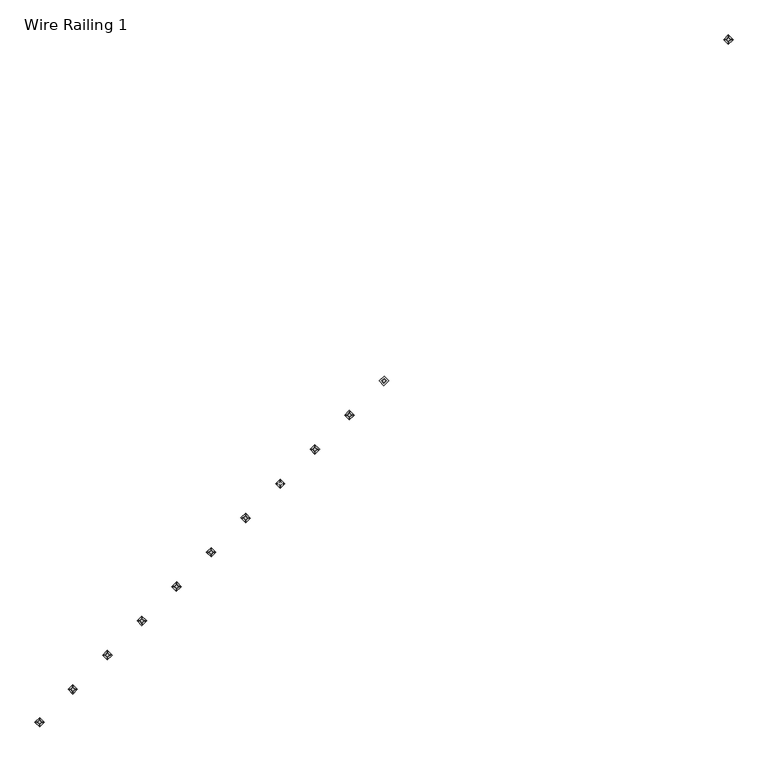
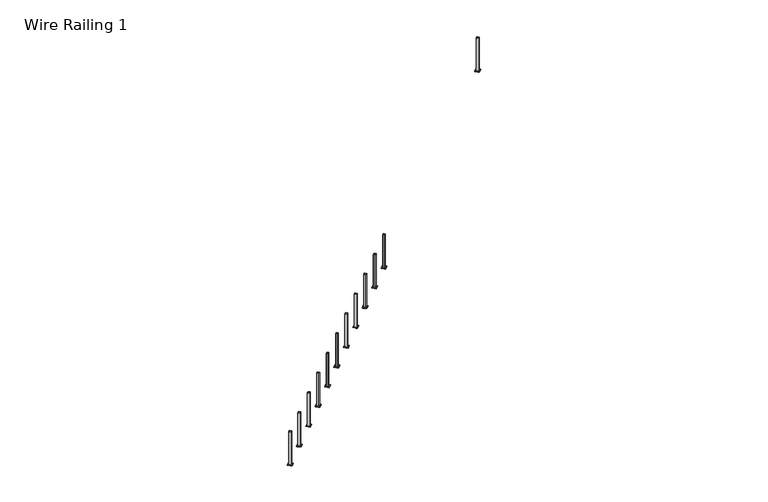
"""IFC4 building model written with IfcOpenShell, lengths in millimetres: railing geometry, Wire Railing 1."""

from ifc_helpers import new_model, si_unit, point, frame, frame_2d, origin, place, context, project, spatial, polyline, circle_curve, trimmed, segment, composite_curve, outline, extrude, source, transform, mapped, element, save


def wire_railing_1_32efedd6(model_context):
    return source(origin(), model_context, "Body", "SweptSolid", [
        extrude(outline(polyline([(39073.6633183, 30885.6288927), (39163.8685639, 30975.0269557), (39253.2666269, 30884.82171), (39163.0613812, 30795.4236471), (39073.6633183, 30885.6288927)])), frame((0.0, 0.0, 263956.8), z_axis=(0.0, 0.0, 1.0), x_axis=(1.0, 0.0, 0.0)), (0.0, 0.0, 1.0), 6.35),
        extrude(outline(polyline([(39120.8091868, 30885.4170073), (39163.6566785, 30927.8810871), (39206.1207584, 30885.0335955), (39163.2732667, 30842.5695156), (39120.8091868, 30885.4170073)]), holes=[polyline([(39129.7893522, 30885.3766481), (39163.3136258, 30851.549681), (39197.1405929, 30885.0739546), (39163.6163193, 30918.9009217), (39129.7893522, 30885.3766481)])]), frame((0.0, 0.0, 263956.8), z_axis=(0.0, 0.0, 1.0), x_axis=(1.0, 0.0, 0.0)), (0.0, 0.0, 1.0), 1047.75),
        extrude(outline(composite_curve([segment(trimmed(circle_curve(frame_2d((38502.5370002, 30167.6303323)), 6.35), [point((38507.0069034, 30163.12007))], [point((38498.0670971, 30172.1405946))], False, "CARTESIAN"), True, "CONTINUOUS"), segment(trimmed(circle_curve(frame_2d((38502.5370002, 30167.6303323)), 6.35), [point((38498.0670971, 30172.1405946))], [point((38507.0069034, 30163.12007))], False, "CARTESIAN"), True, "CONTINUOUS")], self_intersect=False)), frame((0.0, 0.0, 263956.8), z_axis=(0.0, 0.0, 1.0), x_axis=(1.0, 0.0, 0.0)), (0.0, 0.0, 1.0), 12.7),
        extrude(outline(composite_curve([segment(trimmed(circle_curve(frame_2d((38439.9583562, 30230.7740042)), 6.35), [point((38444.4282593, 30226.263742))], [point((38435.488453, 30235.2842665))], False, "CARTESIAN"), True, "CONTINUOUS"), segment(trimmed(circle_curve(frame_2d((38439.9583562, 30230.7740042)), 6.35), [point((38435.488453, 30235.2842665))], [point((38444.4282593, 30226.263742))], False, "CARTESIAN"), True, "CONTINUOUS")], self_intersect=False)), frame((0.0, 0.0, 263956.8), z_axis=(0.0, 0.0, 1.0), x_axis=(1.0, 0.0, 0.0)), (0.0, 0.0, 1.0), 12.7),
        extrude(outline(composite_curve([segment(trimmed(circle_curve(frame_2d((38565.6806722, 30230.2089763)), 6.35), [point((38570.1505753, 30225.6987141))], [point((38561.210769, 30234.7192386))], False, "CARTESIAN"), True, "CONTINUOUS"), segment(trimmed(circle_curve(frame_2d((38565.6806722, 30230.2089763)), 6.35), [point((38561.210769, 30234.7192386))], [point((38570.1505753, 30225.6987141))], False, "CARTESIAN"), True, "CONTINUOUS")], self_intersect=False)), frame((0.0, 0.0, 263956.8), z_axis=(0.0, 0.0, 1.0), x_axis=(1.0, 0.0, 0.0)), (0.0, 0.0, 1.0), 12.7),
        extrude(outline(composite_curve([segment(trimmed(circle_curve(frame_2d((38503.1020281, 30293.3526483)), 6.35), [point((38507.5719313, 30288.842386))], [point((38498.632125, 30297.8629106))], False, "CARTESIAN"), True, "CONTINUOUS"), segment(trimmed(circle_curve(frame_2d((38503.1020281, 30293.3526483)), 6.35), [point((38498.632125, 30297.8629106))], [point((38507.5719313, 30288.842386))], False, "CARTESIAN"), True, "CONTINUOUS")], self_intersect=False)), frame((0.0, 0.0, 263956.8), z_axis=(0.0, 0.0, 1.0), x_axis=(1.0, 0.0, 0.0)), (0.0, 0.0, 1.0), 12.7),
        extrude(outline(polyline([(38413.0178599, 30230.8950817), (38503.2231055, 30320.2931446), (38592.6211685, 30230.0878989), (38502.4159228, 30140.689836), (38413.0178599, 30230.8950817)])), frame((0.0, 0.0, 263956.8), z_axis=(0.0, 0.0, 1.0), x_axis=(1.0, 0.0, 0.0)), (0.0, 0.0, 1.0), 6.35),
        extrude(outline(polyline([(38460.1637284, 30230.6831962), (38503.0112201, 30273.1472761), (38545.4753, 30230.2997844), (38502.6278083, 30187.8357045), (38460.1637284, 30230.6831962)]), holes=[polyline([(38469.1438938, 30230.6428371), (38502.6681674, 30196.8158699), (38536.4951345, 30230.3401435), (38502.9708609, 30264.1671107), (38469.1438938, 30230.6428371)])]), frame((0.0, 0.0, 263956.8), z_axis=(0.0, 0.0, 1.0), x_axis=(1.0, 0.0, 0.0)), (0.0, 0.0, 1.0), 1047.75),
        extrude(outline(composite_curve([segment(trimmed(circle_curve(frame_2d((37841.8915418, 29512.8965212)), 6.35), [point((37846.361445, 29508.3862589))], [point((37837.4216387, 29517.4067835))], False, "CARTESIAN"), True, "CONTINUOUS"), segment(trimmed(circle_curve(frame_2d((37841.8915418, 29512.8965212)), 6.35), [point((37837.4216387, 29517.4067835))], [point((37846.361445, 29508.3862589))], False, "CARTESIAN"), True, "CONTINUOUS")], self_intersect=False)), frame((0.0, 0.0, 263956.8), z_axis=(0.0, 0.0, 1.0), x_axis=(1.0, 0.0, 0.0)), (0.0, 0.0, 1.0), 12.7),
        extrude(outline(composite_curve([segment(trimmed(circle_curve(frame_2d((37779.3128978, 29576.0401932)), 6.35), [point((37783.7828009, 29571.5299309))], [point((37774.8429946, 29580.5504555))], False, "CARTESIAN"), True, "CONTINUOUS"), segment(trimmed(circle_curve(frame_2d((37779.3128978, 29576.0401932)), 6.35), [point((37774.8429946, 29580.5504555))], [point((37783.7828009, 29571.5299309))], False, "CARTESIAN"), True, "CONTINUOUS")], self_intersect=False)), frame((0.0, 0.0, 263956.8), z_axis=(0.0, 0.0, 1.0), x_axis=(1.0, 0.0, 0.0)), (0.0, 0.0, 1.0), 12.7),
        extrude(outline(composite_curve([segment(trimmed(circle_curve(frame_2d((37905.0352138, 29575.4751653)), 6.35), [point((37909.5051169, 29570.964903))], [point((37900.5653106, 29579.9854276))], False, "CARTESIAN"), True, "CONTINUOUS"), segment(trimmed(circle_curve(frame_2d((37905.0352138, 29575.4751653)), 6.35), [point((37900.5653106, 29579.9854276))], [point((37909.5051169, 29570.964903))], False, "CARTESIAN"), True, "CONTINUOUS")], self_intersect=False)), frame((0.0, 0.0, 263956.8), z_axis=(0.0, 0.0, 1.0), x_axis=(1.0, 0.0, 0.0)), (0.0, 0.0, 1.0), 12.7),
        extrude(outline(composite_curve([segment(trimmed(circle_curve(frame_2d((37842.4565697, 29638.6188372)), 6.35), [point((37846.9264729, 29634.1085749))], [point((37837.9866666, 29643.1290995))], False, "CARTESIAN"), True, "CONTINUOUS"), segment(trimmed(circle_curve(frame_2d((37842.4565697, 29638.6188372)), 6.35), [point((37837.9866666, 29643.1290995))], [point((37846.9264729, 29634.1085749))], False, "CARTESIAN"), True, "CONTINUOUS")], self_intersect=False)), frame((0.0, 0.0, 263956.8), z_axis=(0.0, 0.0, 1.0), x_axis=(1.0, 0.0, 0.0)), (0.0, 0.0, 1.0), 12.7),
        extrude(outline(polyline([(37752.3724015, 29576.1612706), (37842.5776471, 29665.5593335), (37931.9757101, 29575.3540879), (37841.7704644, 29485.9560249), (37752.3724015, 29576.1612706)])), frame((0.0, 0.0, 263956.8), z_axis=(0.0, 0.0, 1.0), x_axis=(1.0, 0.0, 0.0)), (0.0, 0.0, 1.0), 6.35),
        extrude(outline(polyline([(37799.51827, 29575.9493851), (37842.3657617, 29618.413465), (37884.8298416, 29575.5659733), (37841.9823499, 29533.1018934), (37799.51827, 29575.9493851)]), holes=[polyline([(37808.4984354, 29575.909026), (37842.022709, 29542.0820589), (37875.8496761, 29575.6063325), (37842.3254025, 29609.4332996), (37808.4984354, 29575.909026)])]), frame((0.0, 0.0, 263956.8), z_axis=(0.0, 0.0, 1.0), x_axis=(1.0, 0.0, 0.0)), (0.0, 0.0, 1.0), 1047.75),
        extrude(outline(composite_curve([segment(trimmed(circle_curve(frame_2d((37181.2460834, 28858.1627102)), 6.35), [point((37185.7159866, 28853.6524479))], [point((37176.7761803, 28862.6729724))], False, "CARTESIAN"), True, "CONTINUOUS"), segment(trimmed(circle_curve(frame_2d((37181.2460834, 28858.1627102)), 6.35), [point((37176.7761803, 28862.6729724))], [point((37185.7159866, 28853.6524479))], False, "CARTESIAN"), True, "CONTINUOUS")], self_intersect=False)), frame((0.0, 0.0, 263956.8), z_axis=(0.0, 0.0, 1.0), x_axis=(1.0, 0.0, 0.0)), (0.0, 0.0, 1.0), 12.7),
        extrude(outline(composite_curve([segment(trimmed(circle_curve(frame_2d((37118.6674394, 28921.3063821)), 6.35), [point((37123.1373425, 28916.7961198))], [point((37114.1975362, 28925.8166444))], False, "CARTESIAN"), True, "CONTINUOUS"), segment(trimmed(circle_curve(frame_2d((37118.6674394, 28921.3063821)), 6.35), [point((37114.1975362, 28925.8166444))], [point((37123.1373425, 28916.7961198))], False, "CARTESIAN"), True, "CONTINUOUS")], self_intersect=False)), frame((0.0, 0.0, 263956.8), z_axis=(0.0, 0.0, 1.0), x_axis=(1.0, 0.0, 0.0)), (0.0, 0.0, 1.0), 12.7),
        extrude(outline(composite_curve([segment(trimmed(circle_curve(frame_2d((37244.3897554, 28920.7413542)), 6.35), [point((37248.8596585, 28916.2310919))], [point((37239.9198522, 28925.2516165))], False, "CARTESIAN"), True, "CONTINUOUS"), segment(trimmed(circle_curve(frame_2d((37244.3897554, 28920.7413542)), 6.35), [point((37239.9198522, 28925.2516165))], [point((37248.8596585, 28916.2310919))], False, "CARTESIAN"), True, "CONTINUOUS")], self_intersect=False)), frame((0.0, 0.0, 263956.8), z_axis=(0.0, 0.0, 1.0), x_axis=(1.0, 0.0, 0.0)), (0.0, 0.0, 1.0), 12.7),
        extrude(outline(composite_curve([segment(trimmed(circle_curve(frame_2d((37181.8111113, 28983.8850262)), 6.35), [point((37186.2810145, 28979.3747639))], [point((37177.3412082, 28988.3952884))], False, "CARTESIAN"), True, "CONTINUOUS"), segment(trimmed(circle_curve(frame_2d((37181.8111113, 28983.8850262)), 6.35), [point((37177.3412082, 28988.3952884))], [point((37186.2810145, 28979.3747639))], False, "CARTESIAN"), True, "CONTINUOUS")], self_intersect=False)), frame((0.0, 0.0, 263956.8), z_axis=(0.0, 0.0, 1.0), x_axis=(1.0, 0.0, 0.0)), (0.0, 0.0, 1.0), 12.7),
        extrude(outline(polyline([(37091.7269431, 28921.4274595), (37181.9321887, 29010.8255225), (37271.3302517, 28920.6202768), (37181.125006, 28831.2222139), (37091.7269431, 28921.4274595)])), frame((0.0, 0.0, 263956.8), z_axis=(0.0, 0.0, 1.0), x_axis=(1.0, 0.0, 0.0)), (0.0, 0.0, 1.0), 6.35),
        extrude(outline(polyline([(37138.8728116, 28921.2155741), (37181.7203033, 28963.6796539), (37224.1843832, 28920.8321623), (37181.3368915, 28878.3680824), (37138.8728116, 28921.2155741)]), holes=[polyline([(37147.852977, 28921.1752149), (37181.3772506, 28887.3482478), (37215.2042177, 28920.8725214), (37181.6799441, 28954.6994885), (37147.852977, 28921.1752149)])]), frame((0.0, 0.0, 263956.8), z_axis=(0.0, 0.0, 1.0), x_axis=(1.0, 0.0, 0.0)), (0.0, 0.0, 1.0), 1047.75),
        extrude(outline(composite_curve([segment(trimmed(circle_curve(frame_2d((36520.600625, 28203.4288991)), 6.35), [point((36525.0705282, 28198.9186368))], [point((36516.1307219, 28207.9391614))], False, "CARTESIAN"), True, "CONTINUOUS"), segment(trimmed(circle_curve(frame_2d((36520.600625, 28203.4288991)), 6.35), [point((36516.1307219, 28207.9391614))], [point((36525.0705282, 28198.9186368))], False, "CARTESIAN"), True, "CONTINUOUS")], self_intersect=False)), frame((0.0, 0.0, 263956.8), z_axis=(0.0, 0.0, 1.0), x_axis=(1.0, 0.0, 0.0)), (0.0, 0.0, 1.0), 12.7),
        extrude(outline(composite_curve([segment(trimmed(circle_curve(frame_2d((36458.021981, 28266.572571)), 6.35), [point((36462.4918841, 28262.0623088))], [point((36453.5520778, 28271.0828333))], False, "CARTESIAN"), True, "CONTINUOUS"), segment(trimmed(circle_curve(frame_2d((36458.021981, 28266.572571)), 6.35), [point((36453.5520778, 28271.0828333))], [point((36462.4918841, 28262.0623088))], False, "CARTESIAN"), True, "CONTINUOUS")], self_intersect=False)), frame((0.0, 0.0, 263956.8), z_axis=(0.0, 0.0, 1.0), x_axis=(1.0, 0.0, 0.0)), (0.0, 0.0, 1.0), 12.7),
        extrude(outline(composite_curve([segment(trimmed(circle_curve(frame_2d((36583.744297, 28266.0075431)), 6.35), [point((36588.2142001, 28261.4972809))], [point((36579.2743938, 28270.5178054))], False, "CARTESIAN"), True, "CONTINUOUS"), segment(trimmed(circle_curve(frame_2d((36583.744297, 28266.0075431)), 6.35), [point((36579.2743938, 28270.5178054))], [point((36588.2142001, 28261.4972809))], False, "CARTESIAN"), True, "CONTINUOUS")], self_intersect=False)), frame((0.0, 0.0, 263956.8), z_axis=(0.0, 0.0, 1.0), x_axis=(1.0, 0.0, 0.0)), (0.0, 0.0, 1.0), 12.7),
        extrude(outline(composite_curve([segment(trimmed(circle_curve(frame_2d((36521.1656529, 28329.1512151)), 6.35), [point((36525.6355561, 28324.6409528))], [point((36516.6957498, 28333.6614774))], False, "CARTESIAN"), True, "CONTINUOUS"), segment(trimmed(circle_curve(frame_2d((36521.1656529, 28329.1512151)), 6.35), [point((36516.6957498, 28333.6614774))], [point((36525.6355561, 28324.6409528))], False, "CARTESIAN"), True, "CONTINUOUS")], self_intersect=False)), frame((0.0, 0.0, 263956.8), z_axis=(0.0, 0.0, 1.0), x_axis=(1.0, 0.0, 0.0)), (0.0, 0.0, 1.0), 12.7),
        extrude(outline(polyline([(36431.0814847, 28266.6936485), (36521.2867303, 28356.0917114), (36610.6847933, 28265.8864657), (36520.4795476, 28176.4884028), (36431.0814847, 28266.6936485)])), frame((0.0, 0.0, 263956.8), z_axis=(0.0, 0.0, 1.0), x_axis=(1.0, 0.0, 0.0)), (0.0, 0.0, 1.0), 6.35),
        extrude(outline(polyline([(36478.2273532, 28266.481763), (36521.0748449, 28308.9458429), (36563.5389248, 28266.0983512), (36520.6914331, 28223.6342713), (36478.2273532, 28266.481763)]), holes=[polyline([(36487.2075186, 28266.4414039), (36520.7317922, 28232.6144367), (36554.5587593, 28266.1387103), (36521.0344857, 28299.9656775), (36487.2075186, 28266.4414039)])]), frame((0.0, 0.0, 263956.8), z_axis=(0.0, 0.0, 1.0), x_axis=(1.0, 0.0, 0.0)), (0.0, 0.0, 1.0), 1047.75),
        extrude(outline(composite_curve([segment(trimmed(circle_curve(frame_2d((35859.9551666, 27548.695088)), 6.35), [point((35864.4250698, 27544.1848257))], [point((35855.4852635, 27553.2053503))], False, "CARTESIAN"), True, "CONTINUOUS"), segment(trimmed(circle_curve(frame_2d((35859.9551666, 27548.695088)), 6.35), [point((35855.4852635, 27553.2053503))], [point((35864.4250698, 27544.1848257))], False, "CARTESIAN"), True, "CONTINUOUS")], self_intersect=False)), frame((0.0, 0.0, 263956.8), z_axis=(0.0, 0.0, 1.0), x_axis=(1.0, 0.0, 0.0)), (0.0, 0.0, 1.0), 12.7),
        extrude(outline(composite_curve([segment(trimmed(circle_curve(frame_2d((35797.3765226, 27611.83876)), 6.35), [point((35801.8464257, 27607.3284977))], [point((35792.9066194, 27616.3490223))], False, "CARTESIAN"), True, "CONTINUOUS"), segment(trimmed(circle_curve(frame_2d((35797.3765226, 27611.83876)), 6.35), [point((35792.9066194, 27616.3490223))], [point((35801.8464257, 27607.3284977))], False, "CARTESIAN"), True, "CONTINUOUS")], self_intersect=False)), frame((0.0, 0.0, 263956.8), z_axis=(0.0, 0.0, 1.0), x_axis=(1.0, 0.0, 0.0)), (0.0, 0.0, 1.0), 12.7),
        extrude(outline(composite_curve([segment(trimmed(circle_curve(frame_2d((35923.0988386, 27611.2737321)), 6.35), [point((35927.5687417, 27606.7634698))], [point((35918.6289354, 27615.7839944))], False, "CARTESIAN"), True, "CONTINUOUS"), segment(trimmed(circle_curve(frame_2d((35923.0988386, 27611.2737321)), 6.35), [point((35918.6289354, 27615.7839944))], [point((35927.5687417, 27606.7634698))], False, "CARTESIAN"), True, "CONTINUOUS")], self_intersect=False)), frame((0.0, 0.0, 263956.8), z_axis=(0.0, 0.0, 1.0), x_axis=(1.0, 0.0, 0.0)), (0.0, 0.0, 1.0), 12.7),
        extrude(outline(composite_curve([segment(trimmed(circle_curve(frame_2d((35860.5201945, 27674.417404)), 6.35), [point((35864.9900977, 27669.9071417))], [point((35856.0502914, 27678.9276663))], False, "CARTESIAN"), True, "CONTINUOUS"), segment(trimmed(circle_curve(frame_2d((35860.5201945, 27674.417404)), 6.35), [point((35856.0502914, 27678.9276663))], [point((35864.9900977, 27669.9071417))], False, "CARTESIAN"), True, "CONTINUOUS")], self_intersect=False)), frame((0.0, 0.0, 263956.8), z_axis=(0.0, 0.0, 1.0), x_axis=(1.0, 0.0, 0.0)), (0.0, 0.0, 1.0), 12.7),
        extrude(outline(polyline([(35770.4360263, 27611.9598374), (35860.6412719, 27701.3579003), (35950.0393349, 27611.1526547), (35859.8340892, 27521.7545917), (35770.4360263, 27611.9598374)])), frame((0.0, 0.0, 263956.8), z_axis=(0.0, 0.0, 1.0), x_axis=(1.0, 0.0, 0.0)), (0.0, 0.0, 1.0), 6.35),
        extrude(outline(polyline([(35817.5818948, 27611.7479519), (35860.4293865, 27654.2120318), (35902.8934664, 27611.3645401), (35860.0459747, 27568.9004602), (35817.5818948, 27611.7479519)]), holes=[polyline([(35826.5620602, 27611.7075928), (35860.0863338, 27577.8806257), (35893.9133009, 27611.4048993), (35860.3890273, 27645.2318664), (35826.5620602, 27611.7075928)])]), frame((0.0, 0.0, 263956.8), z_axis=(0.0, 0.0, 1.0), x_axis=(1.0, 0.0, 0.0)), (0.0, 0.0, 1.0), 1047.75),
        extrude(outline(composite_curve([segment(trimmed(circle_curve(frame_2d((35199.3097082, 26893.961277)), 6.35), [point((35203.7796114, 26889.4510147))], [point((35194.8398051, 26898.4715392))], False, "CARTESIAN"), True, "CONTINUOUS"), segment(trimmed(circle_curve(frame_2d((35199.3097082, 26893.961277)), 6.35), [point((35194.8398051, 26898.4715392))], [point((35203.7796114, 26889.4510147))], False, "CARTESIAN"), True, "CONTINUOUS")], self_intersect=False)), frame((0.0, 0.0, 263956.8), z_axis=(0.0, 0.0, 1.0), x_axis=(1.0, 0.0, 0.0)), (0.0, 0.0, 1.0), 12.7),
        extrude(outline(composite_curve([segment(trimmed(circle_curve(frame_2d((35136.7310642, 26957.1049489)), 6.35), [point((35141.2009673, 26952.5946866))], [point((35132.261161, 26961.6152112))], False, "CARTESIAN"), True, "CONTINUOUS"), segment(trimmed(circle_curve(frame_2d((35136.7310642, 26957.1049489)), 6.35), [point((35132.261161, 26961.6152112))], [point((35141.2009673, 26952.5946866))], False, "CARTESIAN"), True, "CONTINUOUS")], self_intersect=False)), frame((0.0, 0.0, 263956.8), z_axis=(0.0, 0.0, 1.0), x_axis=(1.0, 0.0, 0.0)), (0.0, 0.0, 1.0), 12.7),
        extrude(outline(composite_curve([segment(trimmed(circle_curve(frame_2d((35262.4533802, 26956.539921)), 6.35), [point((35266.9232833, 26952.0296587))], [point((35257.983477, 26961.0501833))], False, "CARTESIAN"), True, "CONTINUOUS"), segment(trimmed(circle_curve(frame_2d((35262.4533802, 26956.539921)), 6.35), [point((35257.983477, 26961.0501833))], [point((35266.9232833, 26952.0296587))], False, "CARTESIAN"), True, "CONTINUOUS")], self_intersect=False)), frame((0.0, 0.0, 263956.8), z_axis=(0.0, 0.0, 1.0), x_axis=(1.0, 0.0, 0.0)), (0.0, 0.0, 1.0), 12.7),
        extrude(outline(composite_curve([segment(trimmed(circle_curve(frame_2d((35199.8747361, 27019.683593)), 6.35), [point((35204.3446393, 27015.1733307))], [point((35195.404833, 27024.1938552))], False, "CARTESIAN"), True, "CONTINUOUS"), segment(trimmed(circle_curve(frame_2d((35199.8747361, 27019.683593)), 6.35), [point((35195.404833, 27024.1938552))], [point((35204.3446393, 27015.1733307))], False, "CARTESIAN"), True, "CONTINUOUS")], self_intersect=False)), frame((0.0, 0.0, 263956.8), z_axis=(0.0, 0.0, 1.0), x_axis=(1.0, 0.0, 0.0)), (0.0, 0.0, 1.0), 12.7),
        extrude(outline(polyline([(35109.7905679, 26957.2260263), (35199.9958135, 27046.6240893), (35289.3938765, 26956.4188436), (35199.1886308, 26867.0207807), (35109.7905679, 26957.2260263)])), frame((0.0, 0.0, 263956.8), z_axis=(0.0, 0.0, 1.0), x_axis=(1.0, 0.0, 0.0)), (0.0, 0.0, 1.0), 6.35),
        extrude(outline(polyline([(35156.9364364, 26957.0141409), (35199.7839281, 26999.4782207), (35242.248008, 26956.6307291), (35199.4005163, 26914.1666492), (35156.9364364, 26957.0141409)]), holes=[polyline([(35165.9166018, 26956.9737817), (35199.4408754, 26923.1468146), (35233.2678425, 26956.6710882), (35199.7435689, 26990.4980553), (35165.9166018, 26956.9737817)])]), frame((0.0, 0.0, 263956.8), z_axis=(0.0, 0.0, 1.0), x_axis=(1.0, 0.0, 0.0)), (0.0, 0.0, 1.0), 1047.75),
        extrude(outline(composite_curve([segment(trimmed(circle_curve(frame_2d((34538.6642498, 26239.2274659)), 6.35), [point((34543.134153, 26234.7172036))], [point((34534.1943467, 26243.7377282))], False, "CARTESIAN"), True, "CONTINUOUS"), segment(trimmed(circle_curve(frame_2d((34538.6642498, 26239.2274659)), 6.35), [point((34534.1943467, 26243.7377282))], [point((34543.134153, 26234.7172036))], False, "CARTESIAN"), True, "CONTINUOUS")], self_intersect=False)), frame((0.0, 0.0, 263956.8), z_axis=(0.0, 0.0, 1.0), x_axis=(1.0, 0.0, 0.0)), (0.0, 0.0, 1.0), 12.7),
        extrude(outline(composite_curve([segment(trimmed(circle_curve(frame_2d((34476.0856058, 26302.3711378)), 6.35), [point((34480.5555089, 26297.8608756))], [point((34471.6157026, 26306.8814001))], False, "CARTESIAN"), True, "CONTINUOUS"), segment(trimmed(circle_curve(frame_2d((34476.0856058, 26302.3711378)), 6.35), [point((34471.6157026, 26306.8814001))], [point((34480.5555089, 26297.8608756))], False, "CARTESIAN"), True, "CONTINUOUS")], self_intersect=False)), frame((0.0, 0.0, 263956.8), z_axis=(0.0, 0.0, 1.0), x_axis=(1.0, 0.0, 0.0)), (0.0, 0.0, 1.0), 12.7),
        extrude(outline(composite_curve([segment(trimmed(circle_curve(frame_2d((34601.8079218, 26301.8061099)), 6.35), [point((34606.2778249, 26297.2958477))], [point((34597.3380186, 26306.3163722))], False, "CARTESIAN"), True, "CONTINUOUS"), segment(trimmed(circle_curve(frame_2d((34601.8079218, 26301.8061099)), 6.35), [point((34597.3380186, 26306.3163722))], [point((34606.2778249, 26297.2958477))], False, "CARTESIAN"), True, "CONTINUOUS")], self_intersect=False)), frame((0.0, 0.0, 263956.8), z_axis=(0.0, 0.0, 1.0), x_axis=(1.0, 0.0, 0.0)), (0.0, 0.0, 1.0), 12.7),
        extrude(outline(composite_curve([segment(trimmed(circle_curve(frame_2d((34539.2292777, 26364.9497819)), 6.35), [point((34543.6991809, 26360.4395196))], [point((34534.7593746, 26369.4600442))], False, "CARTESIAN"), True, "CONTINUOUS"), segment(trimmed(circle_curve(frame_2d((34539.2292777, 26364.9497819)), 6.35), [point((34534.7593746, 26369.4600442))], [point((34543.6991809, 26360.4395196))], False, "CARTESIAN"), True, "CONTINUOUS")], self_intersect=False)), frame((0.0, 0.0, 263956.8), z_axis=(0.0, 0.0, 1.0), x_axis=(1.0, 0.0, 0.0)), (0.0, 0.0, 1.0), 12.7),
        extrude(outline(polyline([(34449.1451095, 26302.4922153), (34539.3503551, 26391.8902782), (34628.7484181, 26301.6850325), (34538.5431724, 26212.2869696), (34449.1451095, 26302.4922153)])), frame((0.0, 0.0, 263956.8), z_axis=(0.0, 0.0, 1.0), x_axis=(1.0, 0.0, 0.0)), (0.0, 0.0, 1.0), 6.35),
        extrude(outline(polyline([(34496.290978, 26302.2803298), (34539.1384697, 26344.7444097), (34581.6025495, 26301.896918), (34538.7550579, 26259.4328381), (34496.290978, 26302.2803298)]), holes=[polyline([(34505.2711434, 26302.2399707), (34538.795417, 26268.4130035), (34572.6223841, 26301.9372771), (34539.0981105, 26335.7642443), (34505.2711434, 26302.2399707)])]), frame((0.0, 0.0, 263956.8), z_axis=(0.0, 0.0, 1.0), x_axis=(1.0, 0.0, 0.0)), (0.0, 0.0, 1.0), 1047.75),
        extrude(outline(composite_curve([segment(trimmed(circle_curve(frame_2d((33878.0187914, 25584.4936548)), 6.35), [point((33882.4886945, 25579.9833925))], [point((33873.5488883, 25589.0039171))], False, "CARTESIAN"), True, "CONTINUOUS"), segment(trimmed(circle_curve(frame_2d((33878.0187914, 25584.4936548)), 6.35), [point((33873.5488883, 25589.0039171))], [point((33882.4886945, 25579.9833925))], False, "CARTESIAN"), True, "CONTINUOUS")], self_intersect=False)), frame((0.0, 0.0, 263956.8), z_axis=(0.0, 0.0, 1.0), x_axis=(1.0, 0.0, 0.0)), (0.0, 0.0, 1.0), 12.7),
        extrude(outline(composite_curve([segment(trimmed(circle_curve(frame_2d((33815.4401473, 25647.6373268)), 6.35), [point((33819.9100505, 25643.1270645))], [point((33810.9702442, 25652.1475891))], False, "CARTESIAN"), True, "CONTINUOUS"), segment(trimmed(circle_curve(frame_2d((33815.4401473, 25647.6373268)), 6.35), [point((33810.9702442, 25652.1475891))], [point((33819.9100505, 25643.1270645))], False, "CARTESIAN"), True, "CONTINUOUS")], self_intersect=False)), frame((0.0, 0.0, 263956.8), z_axis=(0.0, 0.0, 1.0), x_axis=(1.0, 0.0, 0.0)), (0.0, 0.0, 1.0), 12.7),
        extrude(outline(composite_curve([segment(trimmed(circle_curve(frame_2d((33941.1624634, 25647.0722989)), 6.35), [point((33945.6323665, 25642.5620366))], [point((33936.6925602, 25651.5825612))], False, "CARTESIAN"), True, "CONTINUOUS"), segment(trimmed(circle_curve(frame_2d((33941.1624634, 25647.0722989)), 6.35), [point((33936.6925602, 25651.5825612))], [point((33945.6323665, 25642.5620366))], False, "CARTESIAN"), True, "CONTINUOUS")], self_intersect=False)), frame((0.0, 0.0, 263956.8), z_axis=(0.0, 0.0, 1.0), x_axis=(1.0, 0.0, 0.0)), (0.0, 0.0, 1.0), 12.7),
        extrude(outline(composite_curve([segment(trimmed(circle_curve(frame_2d((33878.5838193, 25710.2159708)), 6.35), [point((33883.0537225, 25705.7057086))], [point((33874.1139162, 25714.7262331))], False, "CARTESIAN"), True, "CONTINUOUS"), segment(trimmed(circle_curve(frame_2d((33878.5838193, 25710.2159708)), 6.35), [point((33874.1139162, 25714.7262331))], [point((33883.0537225, 25705.7057086))], False, "CARTESIAN"), True, "CONTINUOUS")], self_intersect=False)), frame((0.0, 0.0, 263956.8), z_axis=(0.0, 0.0, 1.0), x_axis=(1.0, 0.0, 0.0)), (0.0, 0.0, 1.0), 12.7),
        extrude(outline(polyline([(33788.4996511, 25647.7584042), (33878.7048967, 25737.1564671), (33968.1029597, 25646.9512215), (33877.897714, 25557.5531585), (33788.4996511, 25647.7584042)])), frame((0.0, 0.0, 263956.8), z_axis=(0.0, 0.0, 1.0), x_axis=(1.0, 0.0, 0.0)), (0.0, 0.0, 1.0), 6.35),
        extrude(outline(polyline([(33835.6455196, 25647.5465187), (33878.4930113, 25690.0105986), (33920.9570911, 25647.1631069), (33878.1095995, 25604.699027), (33835.6455196, 25647.5465187)]), holes=[polyline([(33844.625685, 25647.5061596), (33878.1499586, 25613.6791925), (33911.9769257, 25647.2034661), (33878.4526521, 25681.0304332), (33844.625685, 25647.5061596)])]), frame((0.0, 0.0, 263956.8), z_axis=(0.0, 0.0, 1.0), x_axis=(1.0, 0.0, 0.0)), (0.0, 0.0, 1.0), 1047.75),
        extrude(outline(composite_curve([segment(trimmed(circle_curve(frame_2d((33217.373333, 24929.7598438)), 6.35), [point((33221.8432361, 24925.2495815))], [point((33212.9034299, 24934.270106))], False, "CARTESIAN"), True, "CONTINUOUS"), segment(trimmed(circle_curve(frame_2d((33217.373333, 24929.7598438)), 6.35), [point((33212.9034299, 24934.270106))], [point((33221.8432361, 24925.2495815))], False, "CARTESIAN"), True, "CONTINUOUS")], self_intersect=False)), frame((0.0, 0.0, 263956.8), z_axis=(0.0, 0.0, 1.0), x_axis=(1.0, 0.0, 0.0)), (0.0, 0.0, 1.0), 12.7),
        extrude(outline(composite_curve([segment(trimmed(circle_curve(frame_2d((33154.7946889, 24992.9035157)), 6.35), [point((33159.2645921, 24988.3932534))], [point((33150.3247858, 24997.413778))], False, "CARTESIAN"), True, "CONTINUOUS"), segment(trimmed(circle_curve(frame_2d((33154.7946889, 24992.9035157)), 6.35), [point((33150.3247858, 24997.413778))], [point((33159.2645921, 24988.3932534))], False, "CARTESIAN"), True, "CONTINUOUS")], self_intersect=False)), frame((0.0, 0.0, 263956.8), z_axis=(0.0, 0.0, 1.0), x_axis=(1.0, 0.0, 0.0)), (0.0, 0.0, 1.0), 12.7),
        extrude(outline(composite_curve([segment(trimmed(circle_curve(frame_2d((33280.517005, 24992.3384878)), 6.35), [point((33284.9869081, 24987.8282255))], [point((33276.0471018, 24996.8487501))], False, "CARTESIAN"), True, "CONTINUOUS"), segment(trimmed(circle_curve(frame_2d((33280.517005, 24992.3384878)), 6.35), [point((33276.0471018, 24996.8487501))], [point((33284.9869081, 24987.8282255))], False, "CARTESIAN"), True, "CONTINUOUS")], self_intersect=False)), frame((0.0, 0.0, 263956.8), z_axis=(0.0, 0.0, 1.0), x_axis=(1.0, 0.0, 0.0)), (0.0, 0.0, 1.0), 12.7),
        extrude(outline(composite_curve([segment(trimmed(circle_curve(frame_2d((33217.9383609, 25055.4821598)), 6.35), [point((33222.4082641, 25050.9718975))], [point((33213.4684578, 25059.992422))], False, "CARTESIAN"), True, "CONTINUOUS"), segment(trimmed(circle_curve(frame_2d((33217.9383609, 25055.4821598)), 6.35), [point((33213.4684578, 25059.992422))], [point((33222.4082641, 25050.9718975))], False, "CARTESIAN"), True, "CONTINUOUS")], self_intersect=False)), frame((0.0, 0.0, 263956.8), z_axis=(0.0, 0.0, 1.0), x_axis=(1.0, 0.0, 0.0)), (0.0, 0.0, 1.0), 12.7),
        extrude(outline(polyline([(33127.8541927, 24993.0245931), (33218.0594383, 25082.4226561), (33307.4575012, 24992.2174104), (33217.2522556, 24902.8193475), (33127.8541927, 24993.0245931)])), frame((0.0, 0.0, 263956.8), z_axis=(0.0, 0.0, 1.0), x_axis=(1.0, 0.0, 0.0)), (0.0, 0.0, 1.0), 6.35),
        extrude(outline(polyline([(33175.0000612, 24992.8127077), (33217.8475528, 25035.2767876), (33260.3116327, 24992.4292959), (33217.4641411, 24949.965216), (33175.0000612, 24992.8127077)]), holes=[polyline([(33183.9802266, 24992.7723485), (33217.5045002, 24958.9453814), (33251.3314673, 24992.469655), (33217.8071937, 25026.2966221), (33183.9802266, 24992.7723485)])]), frame((0.0, 0.0, 263956.8), z_axis=(0.0, 0.0, 1.0), x_axis=(1.0, 0.0, 0.0)), (0.0, 0.0, 1.0), 1047.75),
        extrude(outline(composite_curve([segment(trimmed(circle_curve(frame_2d((45742.575469, 37342.8828351)), 6.35), [point((45747.0453721, 37338.3725729))], [point((45738.1055658, 37347.3930974))], False, "CARTESIAN"), True, "CONTINUOUS"), segment(trimmed(circle_curve(frame_2d((45742.575469, 37342.8828351)), 6.35), [point((45738.1055658, 37347.3930974))], [point((45747.0453721, 37338.3725729))], False, "CARTESIAN"), True, "CONTINUOUS")], self_intersect=False)), frame((0.0, 0.0, 263956.8), z_axis=(0.0, 0.0, 1.0), x_axis=(1.0, 0.0, 0.0)), (0.0, 0.0, 1.0), 12.7),
        extrude(outline(composite_curve([segment(trimmed(circle_curve(frame_2d((45679.9968249, 37406.0265071)), 6.35), [point((45684.466728, 37401.5162448))], [point((45675.5269218, 37410.5367694))], False, "CARTESIAN"), True, "CONTINUOUS"), segment(trimmed(circle_curve(frame_2d((45679.9968249, 37406.0265071)), 6.35), [point((45675.5269218, 37410.5367694))], [point((45684.466728, 37401.5162448))], False, "CARTESIAN"), True, "CONTINUOUS")], self_intersect=False)), frame((0.0, 0.0, 263956.8), z_axis=(0.0, 0.0, 1.0), x_axis=(1.0, 0.0, 0.0)), (0.0, 0.0, 1.0), 12.7),
        extrude(outline(composite_curve([segment(trimmed(circle_curve(frame_2d((45805.7191409, 37405.4614792)), 6.35), [point((45810.1890441, 37400.9512169))], [point((45801.2492378, 37409.9717415))], False, "CARTESIAN"), True, "CONTINUOUS"), segment(trimmed(circle_curve(frame_2d((45805.7191409, 37405.4614792)), 6.35), [point((45801.2492378, 37409.9717415))], [point((45810.1890441, 37400.9512169))], False, "CARTESIAN"), True, "CONTINUOUS")], self_intersect=False)), frame((0.0, 0.0, 263956.8), z_axis=(0.0, 0.0, 1.0), x_axis=(1.0, 0.0, 0.0)), (0.0, 0.0, 1.0), 12.7),
        extrude(outline(composite_curve([segment(trimmed(circle_curve(frame_2d((45743.1404969, 37468.6051512)), 6.35), [point((45747.6104, 37464.0948889))], [point((45738.6705937, 37473.1154134))], False, "CARTESIAN"), True, "CONTINUOUS"), segment(trimmed(circle_curve(frame_2d((45743.1404969, 37468.6051512)), 6.35), [point((45738.6705937, 37473.1154134))], [point((45747.6104, 37464.0948889))], False, "CARTESIAN"), True, "CONTINUOUS")], self_intersect=False)), frame((0.0, 0.0, 263956.8), z_axis=(0.0, 0.0, 1.0), x_axis=(1.0, 0.0, 0.0)), (0.0, 0.0, 1.0), 12.7),
        extrude(outline(polyline([(45653.0563286, 37406.1475845), (45743.2615743, 37495.5456474), (45832.6596372, 37405.3404018), (45742.4543915, 37315.9423388), (45653.0563286, 37406.1475845)])), frame((0.0, 0.0, 263956.8), z_axis=(0.0, 0.0, 1.0), x_axis=(1.0, 0.0, 0.0)), (0.0, 0.0, 1.0), 6.35),
        extrude(outline(polyline([(45700.2021971, 37405.935699), (45743.0496888, 37448.3997789), (45785.5137687, 37405.5522872), (45742.666277, 37363.0882074), (45700.2021971, 37405.935699)]), holes=[polyline([(45709.1823625, 37405.8953399), (45742.7066361, 37372.0683728), (45776.5336033, 37405.5926464), (45743.0093297, 37439.4196135), (45709.1823625, 37405.8953399)])]), frame((0.0, 0.0, 263956.8), z_axis=(0.0, 0.0, 1.0), x_axis=(1.0, 0.0, 0.0)), (0.0, 0.0, 1.0), 1047.75),
        extrude(outline(composite_curve([segment(trimmed(circle_curve(frame_2d((32583.7894483, 24301.8454516)), 6.35), [point((32588.2593514, 24297.3351893))], [point((32579.3195451, 24306.3557139))], False, "CARTESIAN"), True, "CONTINUOUS"), segment(trimmed(circle_curve(frame_2d((32583.7894483, 24301.8454516)), 6.35), [point((32579.3195451, 24306.3557139))], [point((32588.2593514, 24297.3351893))], False, "CARTESIAN"), True, "CONTINUOUS")], self_intersect=False)), frame((0.0, 0.0, 263956.8), z_axis=(0.0, 0.0, 1.0), x_axis=(1.0, 0.0, 0.0)), (0.0, 0.0, 1.0), 12.7),
        extrude(outline(composite_curve([segment(trimmed(circle_curve(frame_2d((32521.2108042, 24364.9891235)), 6.35), [point((32525.6807074, 24360.4788612))], [point((32516.7409011, 24369.4993858))], False, "CARTESIAN"), True, "CONTINUOUS"), segment(trimmed(circle_curve(frame_2d((32521.2108042, 24364.9891235)), 6.35), [point((32516.7409011, 24369.4993858))], [point((32525.6807074, 24360.4788612))], False, "CARTESIAN"), True, "CONTINUOUS")], self_intersect=False)), frame((0.0, 0.0, 263956.8), z_axis=(0.0, 0.0, 1.0), x_axis=(1.0, 0.0, 0.0)), (0.0, 0.0, 1.0), 12.7),
        extrude(outline(composite_curve([segment(trimmed(circle_curve(frame_2d((32646.9331203, 24364.4240956)), 6.35), [point((32651.4030234, 24359.9138333))], [point((32642.4632171, 24368.9343579))], False, "CARTESIAN"), True, "CONTINUOUS"), segment(trimmed(circle_curve(frame_2d((32646.9331203, 24364.4240956)), 6.35), [point((32642.4632171, 24368.9343579))], [point((32651.4030234, 24359.9138333))], False, "CARTESIAN"), True, "CONTINUOUS")], self_intersect=False)), frame((0.0, 0.0, 263956.8), z_axis=(0.0, 0.0, 1.0), x_axis=(1.0, 0.0, 0.0)), (0.0, 0.0, 1.0), 12.7),
        extrude(outline(composite_curve([segment(trimmed(circle_curve(frame_2d((32584.3544762, 24427.5677676)), 6.35), [point((32588.8243793, 24423.0575053))], [point((32579.8845731, 24432.0780299))], False, "CARTESIAN"), True, "CONTINUOUS"), segment(trimmed(circle_curve(frame_2d((32584.3544762, 24427.5677676)), 6.35), [point((32579.8845731, 24432.0780299))], [point((32588.8243793, 24423.0575053))], False, "CARTESIAN"), True, "CONTINUOUS")], self_intersect=False)), frame((0.0, 0.0, 263956.8), z_axis=(0.0, 0.0, 1.0), x_axis=(1.0, 0.0, 0.0)), (0.0, 0.0, 1.0), 12.7),
        extrude(outline(polyline([(32494.270308, 24365.1102009), (32584.4755536, 24454.5082639), (32673.8736165, 24364.3030182), (32583.6683709, 24274.9049553), (32494.270308, 24365.1102009)])), frame((0.0, 0.0, 263956.8), z_axis=(0.0, 0.0, 1.0), x_axis=(1.0, 0.0, 0.0)), (0.0, 0.0, 1.0), 6.35),
        extrude(outline(polyline([(32541.4161765, 24364.8983155), (32584.2636681, 24407.3623954), (32626.727748, 24364.5149037), (32583.8802564, 24322.0508238), (32541.4161765, 24364.8983155)]), holes=[polyline([(32550.3963419, 24364.8579563), (32583.9206155, 24331.0309892), (32617.7475826, 24364.5552628), (32584.223309, 24398.3822299), (32550.3963419, 24364.8579563)])]), frame((0.0, 0.0, 263956.8), z_axis=(0.0, 0.0, 1.0), x_axis=(1.0, 0.0, 0.0)), (0.0, 0.0, 1.0), 1047.75),
    ])


if __name__ == "__main__":
    model = new_model("IFC4")
    model_context = context("Model", 3, world=origin())
    ifc_project = project(units=[si_unit("LENGTHUNIT", "METRE", prefix="MILLI")], contexts=[model_context])
    site = spatial("IfcSite", under=ifc_project)
    building = spatial("IfcBuilding", under=site)
    placement = place(None, origin())
    wire_railing_1_shape = wire_railing_1_32efedd6(model_context)
    element("IfcRailing", 1, ObjectType="Wire Railing 1", at=placement, inside=building, context=model_context, shape_type="MappedRepresentation", body=[
        mapped(wire_railing_1_shape, transform((0.0, 0.0, 0.0), x_axis=(1.0, 0.0, 0.0), y_axis=(0.0, 1.0, 0.0), z_axis=(0.0, 0.0, 1.0))),
    ])
    save(model, "model.ifc")

# Revit data of these elements
# Element 1 (IfcRailing, "Wire Railing 1")
#   Materials on its faces: "WIRE RAILING"
# Materials
#   "WIRE RAILING": class "Metal", colour RGB 244 244 244, transparency 0, Manufacturer = "Kawneer", URL = "http://www.kawneer.com/kawneer/north_america/en/home.asp", Cost = 0
